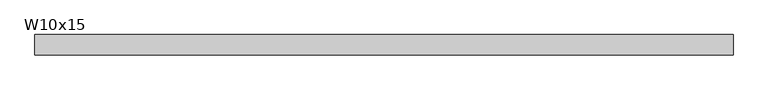
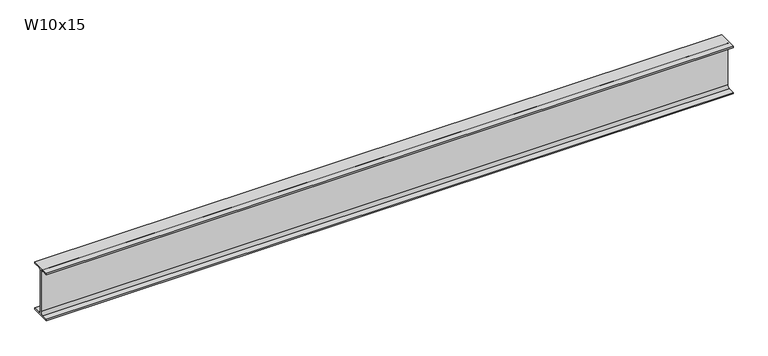
"""IFC4 building model written with IfcOpenShell, lengths in millimetres: beam geometry, RME W-Wide Flange : W10x15."""

from ifc_helpers import new_model, si_unit, point, frame, frame_2d, origin, place, context, project, spatial, polyline, circle_curve, trimmed, segment, composite_curve, outline, extrude, source, transform, mapped, element, save


def w10x15_82c51610(model_context):
    return source(origin(), model_context, "Body", "SweptSolid", [
        extrude(outline(composite_curve([segment(polyline([(50.8, -120.142), (50.8, -127.0), (-50.8, -127.0), (-50.8, -120.142), (-16.7005, -120.142)]), True, "CONTINUOUS"), segment(trimmed(circle_curve(frame_2d((-16.7005, -106.3625)), 13.7795), [point((-16.7005, -120.142))], [point((-2.921, -106.3625))], True, "CARTESIAN"), True, "CONTINUOUS"), segment(polyline([(-2.921, -106.3625), (-2.921, 106.3625)]), True, "CONTINUOUS"), segment(trimmed(circle_curve(frame_2d((-16.7005, 106.3625)), 13.7795), [point((-2.921, 106.3625))], [point((-16.7005, 120.142))], True, "CARTESIAN"), True, "CONTINUOUS"), segment(polyline([(-16.7005, 120.142), (-50.8, 120.142), (-50.8, 127.0), (50.8, 127.0), (50.8, 120.142), (16.7005, 120.142)]), True, "CONTINUOUS"), segment(trimmed(circle_curve(frame_2d((16.7005, 106.3625)), 13.7795), [point((16.7005, 120.142))], [point((2.921, 106.3625))], True, "CARTESIAN"), True, "CONTINUOUS"), segment(polyline([(2.921, 106.3625), (2.921, -106.3625)]), True, "CONTINUOUS"), segment(trimmed(circle_curve(frame_2d((16.7005, -106.3625)), 13.7795), [point((2.921, -106.3625))], [point((16.7005, -120.142))], True, "CARTESIAN"), True, "CONTINUOUS"), segment(polyline([(16.7005, -120.142), (50.8, -120.142)]), True, "CONTINUOUS")], self_intersect=False)), frame((-1739.9, 0.0, 0.0), z_axis=(1.0, 0.0, 0.0), x_axis=(0.0, 1.0, 0.0)), (0.0, 0.0, 1.0), 3479.8),
    ])


if __name__ == "__main__":
    model = new_model("IFC4")
    model_context = context("Model", 3, world=origin())
    ifc_project = project(units=[si_unit("LENGTHUNIT", "METRE", prefix="MILLI")], contexts=[model_context])
    site = spatial("IfcSite", under=ifc_project)
    building = spatial("IfcBuilding", under=site)
    placement = place(None, origin())
    w10x15_shape = w10x15_82c51610(model_context)
    element("IfcBeam", 1, ObjectType="RME W-Wide Flange : W10x15", at=placement, inside=building, context=model_context, shape_type="MappedRepresentation", body=[
        mapped(w10x15_shape, transform((0.0, 0.0, 0.0), x_axis=(1.0, 0.0, 0.0), y_axis=(0.0, 1.0, 0.0), z_axis=(0.0, 0.0, 1.0))),
    ])
    save(model, "model.ifc")

# Revit data of these elements
# Type "RME W-Wide Flange : W10x15"
#   WELD P [instance default] = ""
#   WELD LE [instance default] = ""
#   WELD D [instance default] = ""
#   TOP SECTION SIZE [instance default] = ""
#   TOP SECTION LENGTH [instance default] = ""
#   REMARKS [instance default] = ""
#   REINF TYPE [instance default] = ""
#   Nominal Size = "W24"
#   End Bearing Capacity [instance default] = ""
#   BOT SECTION SIZE [instance default] = ""
#   BOT SECTION LENGTH [instance default] = ""
#   Assembly Code = "B10"
#   W = 15
#   Start Extension Calculation [instance default] = 10' - 0"
#   Start Extension [instance default] = -0' - 0 1/2"
#   End Extension Calculation [instance default] = 10' - 0"
#   End Extension [instance default] = -0' - 0 1/2"
#   Length [instance default] = 5' - 0"
#   bf = 0' - 4"
#   d = 0' - 10"
#   k = 0' - 0 13/16"
#   k2 = 0' - 0.5425"
#   tf = 0' - 0.27"
#   tw = 0' - 0.23"
#   A = 0.030625 SF
#   Structural Material [instance default] = Metal - Steel - ASTM A992
# Element 1 (IfcBeam, "RME W-Wide Flange : W10x15")
#   Length = 11' - 5"
#   Materials on its faces: "Metal - Steel - ASTM A992"
# Materials
#   "Metal - Steel - ASTM A992": class "Metal", colour RGB 255 128 0, transparency 0
